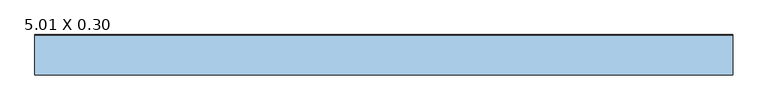
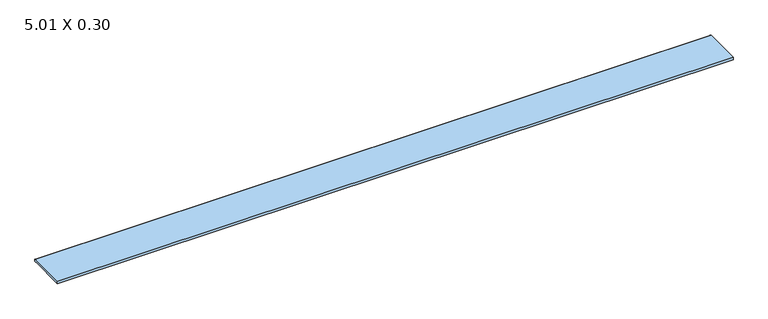
"""IFC4 building model written with IfcOpenShell, lengths in millimetres: window geometry, .CC_ND 300_PEDRA_PEITORIL RETO : 5.01 X 0.30."""

import ifcopenshell
import ifcopenshell.guid

model = None  # the IFC model being written
_history = None  # IfcOwnerHistory: only IFC2X3 demands one
_inside = {}  # id of a spatial element -> (the spatial element, [elements in it])
_under = {}  # id of a project, library or spatial element -> (it, [spatial elements below it])
_declared = {}  # id of a project -> (the project, [libraries it declares])
_typed = {}  # id of a type object -> (the type object, [elements of that type])
_made_of = {}  # id of a material, layer set ... -> (it, [elements and type objects made of it])


def new_model(schema):
    """Start an empty IFC model of exactly this schema.

    Asked for "IFC4X3", IfcOpenShell would pick the latest addendum, in which some entities
    have other attributes; the version numbers below select the first issue.
    IFC2X3 requires an IfcOwnerHistory on every rooted entity: one is made here for all.
    """
    global model, _history
    if schema == "IFC4X3":
        model = ifcopenshell.file(schema_version=(4, 3, 0, 0))
    else:
        model = ifcopenshell.file(schema=schema)
    _inside.clear()
    _under.clear()
    _declared.clear()
    _typed.clear()
    _made_of.clear()
    _history = None
    if model.schema == "IFC2X3":
        org = make("IfcOrganization", Name="unknown")
        user = make(
            "IfcPersonAndOrganization",
            ThePerson=make("IfcPerson", FamilyName="unknown"),
            TheOrganization=org,
        )
        app = make(
            "IfcApplication",
            ApplicationDeveloper=org,
            Version="unknown",
            ApplicationFullName="unknown",
            ApplicationIdentifier="unknown",
        )
        _history = make(
            "IfcOwnerHistory",
            OwningUser=user,
            OwningApplication=app,
            ChangeAction="ADDED",
            CreationDate=0,
        )
    return model


def make(cls, **values):
    """One entity of the class cls with the attributes given. An attribute that is None is left unset."""
    return model.create_entity(
        cls, **{name: value for name, value in values.items() if value is not None}
    )


def rooted(cls, **values):
    """An entity with a GlobalId (a new one), such as an element, a storey or a relation."""
    return make(cls, GlobalId=ifcopenshell.guid.new(), OwnerHistory=_history, **values)


def si_unit(unit_type, name, prefix=None):
    """IfcSIUnit, for example si_unit("LENGTHUNIT", "METRE", prefix="MILLI")."""
    return make("IfcSIUnit", UnitType=unit_type, Prefix=prefix, Name=name)


def assignment(units):
    """IfcUnitAssignment: the units of a project."""
    return None if units is None else make("IfcUnitAssignment", Units=units)


def point(xyz):
    """IfcCartesianPoint."""
    return None if xyz is None else make("IfcCartesianPoint", Coordinates=xyz)


def direction(xyz):
    """IfcDirection."""
    return None if xyz is None else make("IfcDirection", DirectionRatios=xyz)


def frame(location, z_axis=None, x_axis=None):
    """IfcAxis2Placement3D, a coordinate frame: its origin and axes. An axis left out is left unset."""
    return make(
        "IfcAxis2Placement3D",
        Location=point(location),
        Axis=direction(z_axis),
        RefDirection=direction(x_axis),
    )


def frame_2d(location, x_axis=None):
    """IfcAxis2Placement2D, a coordinate frame in the plane: its origin and x axis."""
    return make(
        "IfcAxis2Placement2D", Location=point(location), RefDirection=direction(x_axis)
    )


def origin():
    """The frame at (0, 0, 0) with its axes left unset."""
    return frame((0.0, 0.0, 0.0))


def place(relative_to, where):
    """IfcLocalPlacement: puts the frame where relative to a parent placement (None: the world)."""
    return make(
        "IfcLocalPlacement", PlacementRelTo=relative_to, RelativePlacement=where
    )


def context(
    kind, dimensions, precision=None, world=None, true_north=None, identifier=None
):
    """IfcGeometricRepresentationContext, for example the 3D "Model" context."""
    return make(
        "IfcGeometricRepresentationContext",
        ContextIdentifier=identifier,
        ContextType=kind,
        CoordinateSpaceDimension=dimensions,
        Precision=precision,
        WorldCoordinateSystem=world,
        TrueNorth=true_north,
    )


def project(units=None, contexts=None):
    """IfcProject with its units and contexts."""
    return rooted(
        "IfcProject",
        Name="project",
        RepresentationContexts=contexts,
        UnitsInContext=assignment(units),
    )


def spatial(cls, under=None, at=None, **own):
    """A site, building, storey or space (cls), placed at a placement, below another one or the project."""
    s = rooted(cls, ObjectPlacement=at, **own)
    if under is not None:
        _under.setdefault(under.id(), (under, []))[1].append(s)
    return s


def polyline(points):
    """IfcPolyline through the points."""
    return make("IfcPolyline", Points=[point(p) for p in points])


def circle_curve(where, radius):
    """IfcCircle in the frame where."""
    return make("IfcCircle", Position=where, Radius=radius)


def trimmed(basis, trim1, trim2, sense, master):
    """IfcTrimmedCurve: the piece of a basis curve between two trims."""
    return make(
        "IfcTrimmedCurve",
        BasisCurve=basis,
        Trim1=trim1,
        Trim2=trim2,
        SenseAgreement=sense,
        MasterRepresentation=master,
    )


def segment(curve, same_sense, transition):
    """IfcCompositeCurveSegment."""
    return make(
        "IfcCompositeCurveSegment",
        Transition=transition,
        SameSense=same_sense,
        ParentCurve=curve,
    )


def composite_curve(segments, self_intersect=None):
    """IfcCompositeCurve: segments joined end to end."""
    return make("IfcCompositeCurve", Segments=segments, SelfIntersect=self_intersect)


def outline(outer, holes=None, kind="AREA"):
    """IfcArbitraryClosedProfileDef: a profile drawn as a closed curve; with holes, ...WithVoids."""
    if holes is None:
        return make("IfcArbitraryClosedProfileDef", ProfileType=kind, OuterCurve=outer)
    return make(
        "IfcArbitraryProfileDefWithVoids",
        ProfileType=kind,
        OuterCurve=outer,
        InnerCurves=holes,
    )


def extrude(swept, where, along, depth):
    """IfcExtrudedAreaSolid: the profile swept, set in the frame where, extruded along a direction by depth."""
    return make(
        "IfcExtrudedAreaSolid",
        SweptArea=swept,
        Position=where,
        ExtrudedDirection=direction(along),
        Depth=depth,
    )


def shape(context_of_items, identifier, shape_type, items):
    """IfcShapeRepresentation: the items that make up one representation, for example the "Body"."""
    return make(
        "IfcShapeRepresentation",
        ContextOfItems=context_of_items,
        RepresentationIdentifier=identifier,
        RepresentationType=shape_type,
        Items=items,
    )


def source(mapping_origin, context_of_items, identifier, shape_type, items):
    """IfcRepresentationMap: a shape defined once, which mapped items show again and again."""
    return make(
        "IfcRepresentationMap",
        MappingOrigin=mapping_origin,
        MappedRepresentation=shape(context_of_items, identifier, shape_type, items),
    )


def transform(
    local_origin,
    x_axis=None,
    y_axis=None,
    z_axis=None,
    scale=None,
    scale2=None,
    scale3=None,
    uniform=True,
):
    """IfcCartesianTransformationOperator3D, or its non-uniform kind. x_axis, y_axis, z_axis: its Axis1, 2, 3."""
    if uniform:
        return make(
            "IfcCartesianTransformationOperator3D",
            Axis1=direction(x_axis),
            Axis2=direction(y_axis),
            LocalOrigin=point(local_origin),
            Scale=scale,
            Axis3=direction(z_axis),
        )
    return make(
        "IfcCartesianTransformationOperator3DnonUniform",
        Axis1=direction(x_axis),
        Axis2=direction(y_axis),
        LocalOrigin=point(local_origin),
        Scale=scale,
        Axis3=direction(z_axis),
        Scale2=scale2,
        Scale3=scale3,
    )


def mapped(mapping_source, mapping_target):
    """IfcMappedItem: shows the shape of a source again, moved by a transform."""
    return make(
        "IfcMappedItem", MappingSource=mapping_source, MappingTarget=mapping_target
    )


def made_of(thing, what):
    """Note that an element or type object is made of a material, layer set ...; save() writes the relation."""
    if what is not None:
        _made_of.setdefault(what.id(), (what, []))[1].append(thing)
    return thing


def element(
    cls,
    number,
    at=None,
    inside=None,
    cuts=None,
    type_object=None,
    material=None,
    context=None,
    identifier="Body",
    shape_type=None,
    held_by="IfcProductDefinitionShape",
    body=None,
    shapes=None,
    **own,
):
    """One element of the class cls, such as IfcWall. Its Tag is "e" and its number.

    at: its placement. inside: the storey or other place that contains it. cuts: it is an
    opening in that element (IfcRelVoidsElement). A single representation is given by context,
    identifier, shape_type and body (its items); several are given by shapes. held_by: the class
    of the entity that holds the representations. save() writes the other relations.
    """
    e = rooted(cls, Tag="e%d" % number, ObjectPlacement=at, **own)
    if body is not None:
        shapes = [shape(context, identifier, shape_type, body)]
    if shapes is not None:
        e.Representation = make(held_by, Representations=shapes)
    if inside is not None:
        _inside.setdefault(inside.id(), (inside, []))[1].append(e)
    if cuts is not None:
        rooted(
            "IfcRelVoidsElement", RelatingBuildingElement=cuts, RelatedOpeningElement=e
        )
    if type_object is not None:
        _typed.setdefault(type_object.id(), (type_object, []))[1].append(e)
    return made_of(e, material)


def aggregate(whole, parts):
    """IfcRelAggregates: a whole, such as a stair, and the parts it consists of."""
    return rooted("IfcRelAggregates", RelatingObject=whole, RelatedObjects=parts)


def save(model, path):
    """Write the relations noted so far, then the file.

    IfcRelAggregates (storeys below a building ...), IfcRelContainedInSpatialStructure (elements
    in a storey), IfcRelDefinesByType, IfcRelAssociatesMaterial and IfcRelDeclares: one each for
    every whole, place, type object, material and project.
    """
    for whole, parts in _under.values():
        aggregate(whole, parts)
    for where, things in _inside.values():
        rooted(
            "IfcRelContainedInSpatialStructure",
            RelatedElements=things,
            RelatingStructure=where,
        )
    for kind, things in _typed.values():
        rooted("IfcRelDefinesByType", RelatedObjects=things, RelatingType=kind)
    for what, things in _made_of.values():
        rooted("IfcRelAssociatesMaterial", RelatedObjects=things, RelatingMaterial=what)
    for by, libraries in _declared.values():
        rooted("IfcRelDeclares", RelatingContext=by, RelatedDefinitions=libraries)
    model.write(path)


def window_5_01_x_0_30_29a636ee(model_context):
    return source(origin(), model_context, "Body", "SweptSolid", [
        extrude(outline(composite_curve([segment(polyline([(144.4083081, 1480.0), (-129.9, 1480.0), (-129.9, 1500.0), (153.2808343, 1500.0)]), True, "CONTINUOUS"), segment(trimmed(circle_curve(frame_2d((153.2808343, 1493.3808343)), 6.6191657), [point((153.2808343, 1500.0))], [point((159.9, 1493.3808343))], False, "CARTESIAN"), True, "CONTINUOUS"), segment(polyline([(159.9, 1493.3808343), (159.9, 1480.0), (149.1619526, 1480.0), (149.1619526, 1488.1993124), (144.4083081, 1488.1993124), (144.4083081, 1480.0)]), True, "CONTINUOUS")], self_intersect=False)), frame((-2505.0, 0.0, 0.0), z_axis=(1.0, 0.0, 0.0), x_axis=(0.0, 1.0, 0.0)), (0.0, 0.0, 1.0), 5010.0),
    ])


if __name__ == "__main__":
    model = new_model("IFC4")
    model_context = context("Model", 3, world=origin())
    ifc_project = project(units=[si_unit("LENGTHUNIT", "METRE", prefix="MILLI")], contexts=[model_context])
    site = spatial("IfcSite", under=ifc_project)
    building = spatial("IfcBuilding", under=site)
    placement = place(None, origin())
    window_5_01_x_0_30_shape = window_5_01_x_0_30_29a636ee(model_context)
    element("IfcWindow", 1, ObjectType=".CC_ND 300_PEDRA_PEITORIL RETO : 5.01 X 0.30", at=placement, inside=building, context=model_context, shape_type="MappedRepresentation", body=[
        mapped(window_5_01_x_0_30_shape, transform((0.0, 0.0, 0.0), x_axis=(1.0, 0.0, 0.0), y_axis=(0.0, 1.0, 0.0), z_axis=(0.0, 0.0, 1.0))),
    ])
    save(model, "model.ifc")

# Revit data of these elements
# Project information
#   Design Option = "Main Model"
#   Project Status = "Status do projeto"
#   Client Name = "JOÃO MATIAS SOARES"
#   Project Address = "RUA SÉRGIO DIAS, LOTE 30, QUADRA G, MONTE MINEIRO/MG"
#   Project Name = "CONSTRUÇÃO RESIDENCIA UNIFAMILIAR"
#   Project Number = "034/2017"
#   Zona = "ZER - 01"
#   CA Mín = "0.2"
#   CA Básico = "1"
#   CA Máx = "2"
#   TO Máx = "50"
#   Gabarito Máx = "10"
#   TP Mín = "15"
#   Área Total do Terreno = "620.00 m²"
#   Multifamiliar - Vagas Veículos/Pavto = "0"
#   Multifamiliar - Vagas Bicicletas/Pavto = "0"
#   Multifamiliar - % Vagas PNMR = "0"
#   Multifamiliar - % Vagas Motos = "0"
#   Outros - Área p/ 1 Veículo = "0.00 m²"
#   Outros - Área p/ 1 Bicicleta = "0.00 m²"
#   Outros - Área p/ 1 Utilitário = "0.00 m²"
#   Outros - % Vagas PNMR = "0"
#   Outros - % Vagas Motos = "0"
# Type ".CC_ND 300_PEDRA_PEITORIL RETO : 5.01 X 0.30"
#   Type Mark = "71"
#   Largura da pedra [instance default] = 0.26 m
#   Extensão interior peitoril [instance default] = 0.03 m
#   Extensão exterior peitoril [instance default] = 0.03 m
#   Espessura = 0.02 m
#   Comprimento = 5.01 m
#   Altura-padrão do peitoril = 1.48 m
#   Peitoril = .GRANITO_BRANCO_ITAUNAS
#   Rough Width = 0
#   Rough Height = 0
#   Height = 0
#   Wall Closure = (empty or 0)
#   Width = 0
# Element 1 (IfcWindow, ".CC_ND 300_PEDRA_PEITORIL RETO : 5.01 X 0.30")
#   Largura da pedra = 0.2898 m
#   Extensão interior peitoril = 0.00 m
#   Materials on its faces: ".GRANITO_BRANCO_ITAUNAS"
# Materials
#   ".GRANITO_BRANCO_ITAUNAS": class ".CC_PEDRA REVEST.", colour RGB 202 195 174, transparency 0, Description = "Revestimento em granito", Cost = 0
